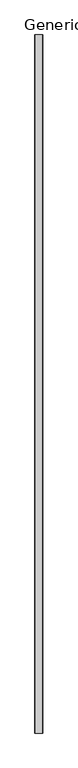
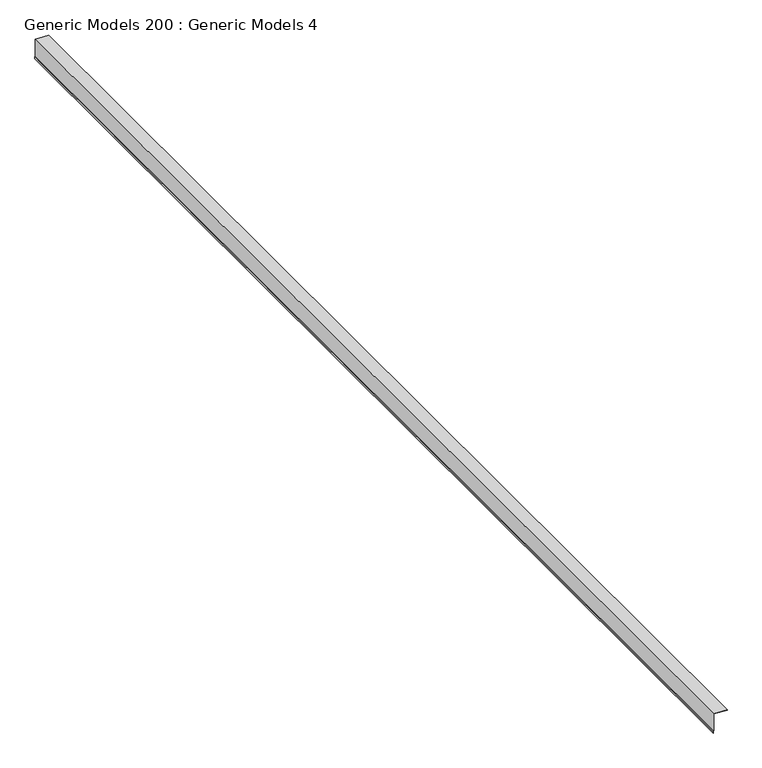
"""IFC4 building model written with IfcOpenShell, lengths in millimetres: proxy geometry, Generic Models 200 : Generic Models 4."""

from ifc_helpers import new_model, si_unit, frame, origin, place, context, project, spatial, polyline, outline, extrude, source, transform, mapped, element, save


def generic_models_200_generic_models_4_d7d1267f(model_context):
    return source(origin(), model_context, "Body", "SweptSolid", [
        extrude(outline(polyline([(126712.1725001, -8349.4098663), (126719.3044406, -8346.8140523), (126931.3921326, -8346.8140523), (126924.8125517, -8188.9041115), (126925.6083721, -8188.9372707), (126932.2196442, -8347.6078023), (126719.4444002, -8347.6078023), (126712.3124596, -8350.2036163), (126693.1385401, -8350.2036163), (126693.1385401, -8349.4098663), (126712.1725001, -8349.4098663)])), frame((0.0, -6864.9230338, 0.0), z_axis=(0.0, 1.0, 0.0), x_axis=(0.0, 0.0, 1.0)), (0.0, 0.0, 1.0), 13919.2),
    ])


if __name__ == "__main__":
    model = new_model("IFC4")
    model_context = context("Model", 3, world=origin())
    ifc_project = project(units=[si_unit("LENGTHUNIT", "METRE", prefix="MILLI")], contexts=[model_context])
    site = spatial("IfcSite", under=ifc_project)
    building = spatial("IfcBuilding", under=site)
    placement = place(None, origin())
    generic_models_200_generic_models_4_shape = generic_models_200_generic_models_4_d7d1267f(model_context)
    element("IfcBuildingElementProxy", 1, Name="Generic Models 200 : Generic Models 4", ObjectType="Generic Models 200 : Generic Models 4", at=placement, inside=building, context=model_context, shape_type="MappedRepresentation", body=[
        mapped(generic_models_200_generic_models_4_shape, transform((0.0, 0.0, 0.0), x_axis=(1.0, 0.0, 0.0), y_axis=(0.0, 1.0, 0.0), z_axis=(0.0, 0.0, 1.0))),
    ])
    save(model, "model.ifc")

# Revit data of these elements
# Element 1 (IfcBuildingElementProxy, "Generic Models 200 : Generic Models 4")
#   Materials on its faces: "_(2) LAYERS NO. 30 ASTM D226 ASPHALT SATURATED ORGANIC FELT"
# Materials
#   "_(2) LAYERS NO. 30 ASTM D226 ASPHALT SATURATED ORGANIC FELT": class "Generic", colour RGB 67 154 161, transparency 0, Cost = 0
